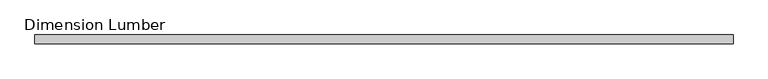
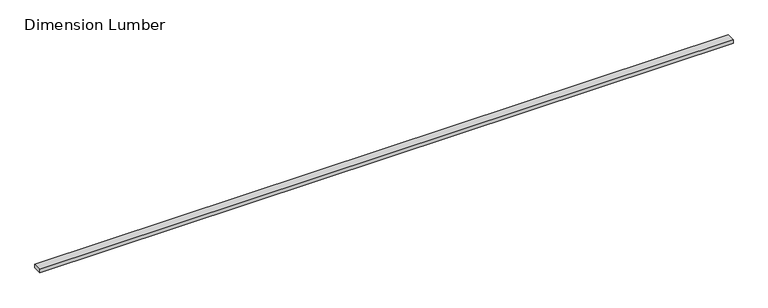
"""IFC4 building model written with IfcOpenShell, lengths in millimetres: beam geometry, Dimension Lumber : Top Supporting Lumbers."""

import ifcopenshell
import ifcopenshell.guid

model = None  # the IFC model being written
_history = None  # IfcOwnerHistory: only IFC2X3 demands one
_inside = {}  # id of a spatial element -> (the spatial element, [elements in it])
_under = {}  # id of a project, library or spatial element -> (it, [spatial elements below it])
_declared = {}  # id of a project -> (the project, [libraries it declares])
_typed = {}  # id of a type object -> (the type object, [elements of that type])
_made_of = {}  # id of a material, layer set ... -> (it, [elements and type objects made of it])


def new_model(schema):
    """Start an empty IFC model of exactly this schema.

    Asked for "IFC4X3", IfcOpenShell would pick the latest addendum, in which some entities
    have other attributes; the version numbers below select the first issue.
    IFC2X3 requires an IfcOwnerHistory on every rooted entity: one is made here for all.
    """
    global model, _history
    if schema == "IFC4X3":
        model = ifcopenshell.file(schema_version=(4, 3, 0, 0))
    else:
        model = ifcopenshell.file(schema=schema)
    _inside.clear()
    _under.clear()
    _declared.clear()
    _typed.clear()
    _made_of.clear()
    _history = None
    if model.schema == "IFC2X3":
        org = make("IfcOrganization", Name="unknown")
        user = make(
            "IfcPersonAndOrganization",
            ThePerson=make("IfcPerson", FamilyName="unknown"),
            TheOrganization=org,
        )
        app = make(
            "IfcApplication",
            ApplicationDeveloper=org,
            Version="unknown",
            ApplicationFullName="unknown",
            ApplicationIdentifier="unknown",
        )
        _history = make(
            "IfcOwnerHistory",
            OwningUser=user,
            OwningApplication=app,
            ChangeAction="ADDED",
            CreationDate=0,
        )
    return model


def make(cls, **values):
    """One entity of the class cls with the attributes given. An attribute that is None is left unset."""
    return model.create_entity(
        cls, **{name: value for name, value in values.items() if value is not None}
    )


def rooted(cls, **values):
    """An entity with a GlobalId (a new one), such as an element, a storey or a relation."""
    return make(cls, GlobalId=ifcopenshell.guid.new(), OwnerHistory=_history, **values)


def si_unit(unit_type, name, prefix=None):
    """IfcSIUnit, for example si_unit("LENGTHUNIT", "METRE", prefix="MILLI")."""
    return make("IfcSIUnit", UnitType=unit_type, Prefix=prefix, Name=name)


def assignment(units):
    """IfcUnitAssignment: the units of a project."""
    return None if units is None else make("IfcUnitAssignment", Units=units)


def point(xyz):
    """IfcCartesianPoint."""
    return None if xyz is None else make("IfcCartesianPoint", Coordinates=xyz)


def direction(xyz):
    """IfcDirection."""
    return None if xyz is None else make("IfcDirection", DirectionRatios=xyz)


def frame(location, z_axis=None, x_axis=None):
    """IfcAxis2Placement3D, a coordinate frame: its origin and axes. An axis left out is left unset."""
    return make(
        "IfcAxis2Placement3D",
        Location=point(location),
        Axis=direction(z_axis),
        RefDirection=direction(x_axis),
    )


def origin():
    """The frame at (0, 0, 0) with its axes left unset."""
    return frame((0.0, 0.0, 0.0))


def place(relative_to, where):
    """IfcLocalPlacement: puts the frame where relative to a parent placement (None: the world)."""
    return make(
        "IfcLocalPlacement", PlacementRelTo=relative_to, RelativePlacement=where
    )


def context(
    kind, dimensions, precision=None, world=None, true_north=None, identifier=None
):
    """IfcGeometricRepresentationContext, for example the 3D "Model" context."""
    return make(
        "IfcGeometricRepresentationContext",
        ContextIdentifier=identifier,
        ContextType=kind,
        CoordinateSpaceDimension=dimensions,
        Precision=precision,
        WorldCoordinateSystem=world,
        TrueNorth=true_north,
    )


def project(units=None, contexts=None):
    """IfcProject with its units and contexts."""
    return rooted(
        "IfcProject",
        Name="project",
        RepresentationContexts=contexts,
        UnitsInContext=assignment(units),
    )


def spatial(cls, under=None, at=None, **own):
    """A site, building, storey or space (cls), placed at a placement, below another one or the project."""
    s = rooted(cls, ObjectPlacement=at, **own)
    if under is not None:
        _under.setdefault(under.id(), (under, []))[1].append(s)
    return s


def polyline(points):
    """IfcPolyline through the points."""
    return make("IfcPolyline", Points=[point(p) for p in points])


def outline(outer, holes=None, kind="AREA"):
    """IfcArbitraryClosedProfileDef: a profile drawn as a closed curve; with holes, ...WithVoids."""
    if holes is None:
        return make("IfcArbitraryClosedProfileDef", ProfileType=kind, OuterCurve=outer)
    return make(
        "IfcArbitraryProfileDefWithVoids",
        ProfileType=kind,
        OuterCurve=outer,
        InnerCurves=holes,
    )


def extrude(swept, where, along, depth):
    """IfcExtrudedAreaSolid: the profile swept, set in the frame where, extruded along a direction by depth."""
    return make(
        "IfcExtrudedAreaSolid",
        SweptArea=swept,
        Position=where,
        ExtrudedDirection=direction(along),
        Depth=depth,
    )


def shape(context_of_items, identifier, shape_type, items):
    """IfcShapeRepresentation: the items that make up one representation, for example the "Body"."""
    return make(
        "IfcShapeRepresentation",
        ContextOfItems=context_of_items,
        RepresentationIdentifier=identifier,
        RepresentationType=shape_type,
        Items=items,
    )


def source(mapping_origin, context_of_items, identifier, shape_type, items):
    """IfcRepresentationMap: a shape defined once, which mapped items show again and again."""
    return make(
        "IfcRepresentationMap",
        MappingOrigin=mapping_origin,
        MappedRepresentation=shape(context_of_items, identifier, shape_type, items),
    )


def transform(
    local_origin,
    x_axis=None,
    y_axis=None,
    z_axis=None,
    scale=None,
    scale2=None,
    scale3=None,
    uniform=True,
):
    """IfcCartesianTransformationOperator3D, or its non-uniform kind. x_axis, y_axis, z_axis: its Axis1, 2, 3."""
    if uniform:
        return make(
            "IfcCartesianTransformationOperator3D",
            Axis1=direction(x_axis),
            Axis2=direction(y_axis),
            LocalOrigin=point(local_origin),
            Scale=scale,
            Axis3=direction(z_axis),
        )
    return make(
        "IfcCartesianTransformationOperator3DnonUniform",
        Axis1=direction(x_axis),
        Axis2=direction(y_axis),
        LocalOrigin=point(local_origin),
        Scale=scale,
        Axis3=direction(z_axis),
        Scale2=scale2,
        Scale3=scale3,
    )


def mapped(mapping_source, mapping_target):
    """IfcMappedItem: shows the shape of a source again, moved by a transform."""
    return make(
        "IfcMappedItem", MappingSource=mapping_source, MappingTarget=mapping_target
    )


def made_of(thing, what):
    """Note that an element or type object is made of a material, layer set ...; save() writes the relation."""
    if what is not None:
        _made_of.setdefault(what.id(), (what, []))[1].append(thing)
    return thing


def element(
    cls,
    number,
    at=None,
    inside=None,
    cuts=None,
    type_object=None,
    material=None,
    context=None,
    identifier="Body",
    shape_type=None,
    held_by="IfcProductDefinitionShape",
    body=None,
    shapes=None,
    **own,
):
    """One element of the class cls, such as IfcWall. Its Tag is "e" and its number.

    at: its placement. inside: the storey or other place that contains it. cuts: it is an
    opening in that element (IfcRelVoidsElement). A single representation is given by context,
    identifier, shape_type and body (its items); several are given by shapes. held_by: the class
    of the entity that holds the representations. save() writes the other relations.
    """
    e = rooted(cls, Tag="e%d" % number, ObjectPlacement=at, **own)
    if body is not None:
        shapes = [shape(context, identifier, shape_type, body)]
    if shapes is not None:
        e.Representation = make(held_by, Representations=shapes)
    if inside is not None:
        _inside.setdefault(inside.id(), (inside, []))[1].append(e)
    if cuts is not None:
        rooted(
            "IfcRelVoidsElement", RelatingBuildingElement=cuts, RelatedOpeningElement=e
        )
    if type_object is not None:
        _typed.setdefault(type_object.id(), (type_object, []))[1].append(e)
    return made_of(e, material)


def aggregate(whole, parts):
    """IfcRelAggregates: a whole, such as a stair, and the parts it consists of."""
    return rooted("IfcRelAggregates", RelatingObject=whole, RelatedObjects=parts)


def save(model, path):
    """Write the relations noted so far, then the file.

    IfcRelAggregates (storeys below a building ...), IfcRelContainedInSpatialStructure (elements
    in a storey), IfcRelDefinesByType, IfcRelAssociatesMaterial and IfcRelDeclares: one each for
    every whole, place, type object, material and project.
    """
    for whole, parts in _under.values():
        aggregate(whole, parts)
    for where, things in _inside.values():
        rooted(
            "IfcRelContainedInSpatialStructure",
            RelatedElements=things,
            RelatingStructure=where,
        )
    for kind, things in _typed.values():
        rooted("IfcRelDefinesByType", RelatedObjects=things, RelatingType=kind)
    for what, things in _made_of.values():
        rooted("IfcRelAssociatesMaterial", RelatedObjects=things, RelatingMaterial=what)
    for by, libraries in _declared.values():
        rooted("IfcRelDeclares", RelatingContext=by, RelatedDefinitions=libraries)
    model.write(path)


def dimension_lumber_96205b60(model_context):
    return source(origin(), model_context, "Body", "SweptSolid", [
        extrude(outline(polyline([(3550.44375, 44.45), (3550.44375, -44.45), (-3550.44375, -44.45), (-3550.44375, 44.45), (3550.44375, 44.45)])), frame((0.0, 0.0, -19.05), z_axis=(0.0, 0.0, 1.0), x_axis=(1.0, 0.0, 0.0)), (0.0, 0.0, 1.0), 38.1),
    ])


if __name__ == "__main__":
    model = new_model("IFC4")
    model_context = context("Model", 3, world=origin())
    ifc_project = project(units=[si_unit("LENGTHUNIT", "METRE", prefix="MILLI")], contexts=[model_context])
    site = spatial("IfcSite", under=ifc_project)
    building = spatial("IfcBuilding", under=site)
    placement = place(None, origin())
    dimension_lumber_shape = dimension_lumber_96205b60(model_context)
    element("IfcBeam", 1, ObjectType="Dimension Lumber : Top Supporting Lumbers", at=placement, inside=building, context=model_context, shape_type="MappedRepresentation", body=[
        mapped(dimension_lumber_shape, transform((0.0, 0.0, 0.0), x_axis=(1.0, 0.0, 0.0), y_axis=(0.0, 1.0, 0.0), z_axis=(0.0, 0.0, 1.0))),
    ])
    save(model, "model.ifc")

# Revit data of these elements
# Type "Dimension Lumber : Top Supporting Lumbers"
#   Assembly Code = "B10"
#   A = 0.0364583 SF
#   Length [instance default] = 5' - 0"
#   b = 0' - 3 1/2"
#   d = 0' - 1 1/2"
#   Structural Material [instance default] = Softwood, Lumber
# Element 1 (IfcBeam, "Dimension Lumber : Top Supporting Lumbers")
#   Structural Material = Douglas Fir #2
#   Materials on its faces: "Douglas Fir #2"
# Materials
#   "Softwood, Lumber": class "Wood", colour RGB 223 192 134, transparency 0, Description = "Pinus Echinata", Cost = 0
#   "Douglas Fir #2": class "Wood", colour RGB 223 192 134, transparency 0, Description = "Pinus Echinata", Cost = 0
